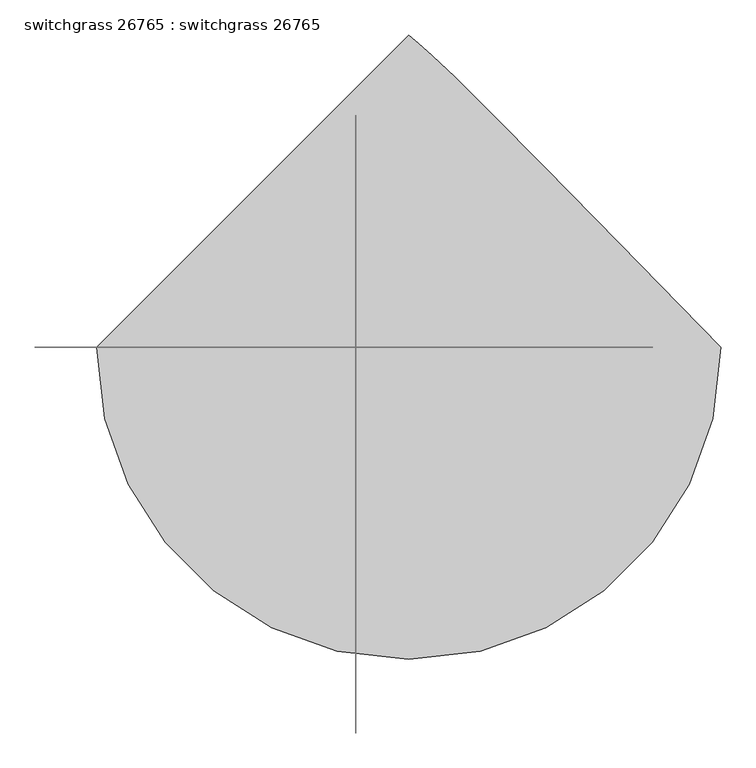
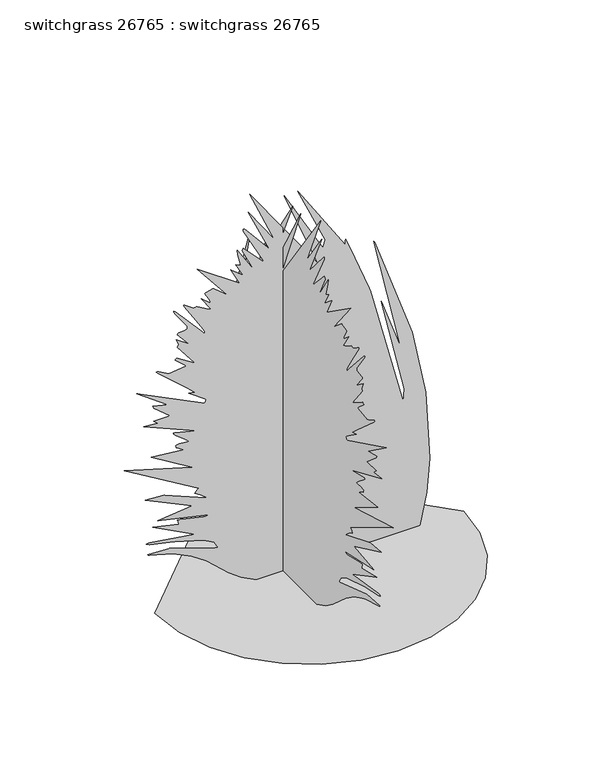
"""IFC4 building model written with IfcOpenShell, lengths in millimetres: proxy geometry, switchgrass 26765 : switchgrass 26765."""

import ifcopenshell
import ifcopenshell.guid

model = None  # the IFC model being written
_history = None  # IfcOwnerHistory: only IFC2X3 demands one
_inside = {}  # id of a spatial element -> (the spatial element, [elements in it])
_under = {}  # id of a project, library or spatial element -> (it, [spatial elements below it])
_declared = {}  # id of a project -> (the project, [libraries it declares])
_typed = {}  # id of a type object -> (the type object, [elements of that type])
_made_of = {}  # id of a material, layer set ... -> (it, [elements and type objects made of it])


def new_model(schema):
    """Start an empty IFC model of exactly this schema.

    Asked for "IFC4X3", IfcOpenShell would pick the latest addendum, in which some entities
    have other attributes; the version numbers below select the first issue.
    IFC2X3 requires an IfcOwnerHistory on every rooted entity: one is made here for all.
    """
    global model, _history
    if schema == "IFC4X3":
        model = ifcopenshell.file(schema_version=(4, 3, 0, 0))
    else:
        model = ifcopenshell.file(schema=schema)
    _inside.clear()
    _under.clear()
    _declared.clear()
    _typed.clear()
    _made_of.clear()
    _history = None
    if model.schema == "IFC2X3":
        org = make("IfcOrganization", Name="unknown")
        user = make(
            "IfcPersonAndOrganization",
            ThePerson=make("IfcPerson", FamilyName="unknown"),
            TheOrganization=org,
        )
        app = make(
            "IfcApplication",
            ApplicationDeveloper=org,
            Version="unknown",
            ApplicationFullName="unknown",
            ApplicationIdentifier="unknown",
        )
        _history = make(
            "IfcOwnerHistory",
            OwningUser=user,
            OwningApplication=app,
            ChangeAction="ADDED",
            CreationDate=0,
        )
    return model


def make(cls, **values):
    """One entity of the class cls with the attributes given. An attribute that is None is left unset."""
    return model.create_entity(
        cls, **{name: value for name, value in values.items() if value is not None}
    )


def rooted(cls, **values):
    """An entity with a GlobalId (a new one), such as an element, a storey or a relation."""
    return make(cls, GlobalId=ifcopenshell.guid.new(), OwnerHistory=_history, **values)


def si_unit(unit_type, name, prefix=None):
    """IfcSIUnit, for example si_unit("LENGTHUNIT", "METRE", prefix="MILLI")."""
    return make("IfcSIUnit", UnitType=unit_type, Prefix=prefix, Name=name)


def assignment(units):
    """IfcUnitAssignment: the units of a project."""
    return None if units is None else make("IfcUnitAssignment", Units=units)


def point(xyz):
    """IfcCartesianPoint."""
    return None if xyz is None else make("IfcCartesianPoint", Coordinates=xyz)


def direction(xyz):
    """IfcDirection."""
    return None if xyz is None else make("IfcDirection", DirectionRatios=xyz)


def frame(location, z_axis=None, x_axis=None):
    """IfcAxis2Placement3D, a coordinate frame: its origin and axes. An axis left out is left unset."""
    return make(
        "IfcAxis2Placement3D",
        Location=point(location),
        Axis=direction(z_axis),
        RefDirection=direction(x_axis),
    )


def origin():
    """The frame at (0, 0, 0) with its axes left unset."""
    return frame((0.0, 0.0, 0.0))


def place(relative_to, where):
    """IfcLocalPlacement: puts the frame where relative to a parent placement (None: the world)."""
    return make(
        "IfcLocalPlacement", PlacementRelTo=relative_to, RelativePlacement=where
    )


def context(
    kind, dimensions, precision=None, world=None, true_north=None, identifier=None
):
    """IfcGeometricRepresentationContext, for example the 3D "Model" context."""
    return make(
        "IfcGeometricRepresentationContext",
        ContextIdentifier=identifier,
        ContextType=kind,
        CoordinateSpaceDimension=dimensions,
        Precision=precision,
        WorldCoordinateSystem=world,
        TrueNorth=true_north,
    )


def project(units=None, contexts=None):
    """IfcProject with its units and contexts."""
    return rooted(
        "IfcProject",
        Name="project",
        RepresentationContexts=contexts,
        UnitsInContext=assignment(units),
    )


def spatial(cls, under=None, at=None, **own):
    """A site, building, storey or space (cls), placed at a placement, below another one or the project."""
    s = rooted(cls, ObjectPlacement=at, **own)
    if under is not None:
        _under.setdefault(under.id(), (under, []))[1].append(s)
    return s


def point_list(points):
    """IfcCartesianPointList2D or 3D."""
    cls = (
        "IfcCartesianPointList2D" if len(points[0]) == 2 else "IfcCartesianPointList3D"
    )
    return make(cls, CoordList=points)


def triangles(points, corners, closed=None, point_numbers=None):
    """IfcTriangulatedFaceSet: each triangle names its three corners, points numbered from 1."""
    return make(
        "IfcTriangulatedFaceSet",
        Coordinates=point_list(points),
        Closed=closed,
        CoordIndex=corners,
        PnIndex=point_numbers,
    )


def shape(context_of_items, identifier, shape_type, items):
    """IfcShapeRepresentation: the items that make up one representation, for example the "Body"."""
    return make(
        "IfcShapeRepresentation",
        ContextOfItems=context_of_items,
        RepresentationIdentifier=identifier,
        RepresentationType=shape_type,
        Items=items,
    )


def source(mapping_origin, context_of_items, identifier, shape_type, items):
    """IfcRepresentationMap: a shape defined once, which mapped items show again and again."""
    return make(
        "IfcRepresentationMap",
        MappingOrigin=mapping_origin,
        MappedRepresentation=shape(context_of_items, identifier, shape_type, items),
    )


def transform(
    local_origin,
    x_axis=None,
    y_axis=None,
    z_axis=None,
    scale=None,
    scale2=None,
    scale3=None,
    uniform=True,
):
    """IfcCartesianTransformationOperator3D, or its non-uniform kind. x_axis, y_axis, z_axis: its Axis1, 2, 3."""
    if uniform:
        return make(
            "IfcCartesianTransformationOperator3D",
            Axis1=direction(x_axis),
            Axis2=direction(y_axis),
            LocalOrigin=point(local_origin),
            Scale=scale,
            Axis3=direction(z_axis),
        )
    return make(
        "IfcCartesianTransformationOperator3DnonUniform",
        Axis1=direction(x_axis),
        Axis2=direction(y_axis),
        LocalOrigin=point(local_origin),
        Scale=scale,
        Axis3=direction(z_axis),
        Scale2=scale2,
        Scale3=scale3,
    )


def mapped(mapping_source, mapping_target):
    """IfcMappedItem: shows the shape of a source again, moved by a transform."""
    return make(
        "IfcMappedItem", MappingSource=mapping_source, MappingTarget=mapping_target
    )


def made_of(thing, what):
    """Note that an element or type object is made of a material, layer set ...; save() writes the relation."""
    if what is not None:
        _made_of.setdefault(what.id(), (what, []))[1].append(thing)
    return thing


def element(
    cls,
    number,
    at=None,
    inside=None,
    cuts=None,
    type_object=None,
    material=None,
    context=None,
    identifier="Body",
    shape_type=None,
    held_by="IfcProductDefinitionShape",
    body=None,
    shapes=None,
    **own,
):
    """One element of the class cls, such as IfcWall. Its Tag is "e" and its number.

    at: its placement. inside: the storey or other place that contains it. cuts: it is an
    opening in that element (IfcRelVoidsElement). A single representation is given by context,
    identifier, shape_type and body (its items); several are given by shapes. held_by: the class
    of the entity that holds the representations. save() writes the other relations.
    """
    e = rooted(cls, Tag="e%d" % number, ObjectPlacement=at, **own)
    if body is not None:
        shapes = [shape(context, identifier, shape_type, body)]
    if shapes is not None:
        e.Representation = make(held_by, Representations=shapes)
    if inside is not None:
        _inside.setdefault(inside.id(), (inside, []))[1].append(e)
    if cuts is not None:
        rooted(
            "IfcRelVoidsElement", RelatingBuildingElement=cuts, RelatedOpeningElement=e
        )
    if type_object is not None:
        _typed.setdefault(type_object.id(), (type_object, []))[1].append(e)
    return made_of(e, material)


def aggregate(whole, parts):
    """IfcRelAggregates: a whole, such as a stair, and the parts it consists of."""
    return rooted("IfcRelAggregates", RelatingObject=whole, RelatedObjects=parts)


def save(model, path):
    """Write the relations noted so far, then the file.

    IfcRelAggregates (storeys below a building ...), IfcRelContainedInSpatialStructure (elements
    in a storey), IfcRelDefinesByType, IfcRelAssociatesMaterial and IfcRelDeclares: one each for
    every whole, place, type object, material and project.
    """
    for whole, parts in _under.values():
        aggregate(whole, parts)
    for where, things in _inside.values():
        rooted(
            "IfcRelContainedInSpatialStructure",
            RelatedElements=things,
            RelatingStructure=where,
        )
    for kind, things in _typed.values():
        rooted("IfcRelDefinesByType", RelatedObjects=things, RelatingType=kind)
    for what, things in _made_of.values():
        rooted("IfcRelAssociatesMaterial", RelatedObjects=things, RelatingMaterial=what)
    for by, libraries in _declared.values():
        rooted("IfcRelDeclares", RelatingContext=by, RelatedDefinitions=libraries)
    model.write(path)


def switchgrass_26765_switchgrass_26765_d4ad6bd8(model_context):
    return source(origin(), model_context, "Body", "Tessellation", [
        triangles([(-459.698612, 0.0, 4.65e-05), (-447.5447391, -105.3326149, 4.65e-05), (-412.9347513, -202.0637927, 4.65e-05), (-358.6347227, -287.4208646, 4.65e-05), (-287.4208646, -358.6372662, 4.65e-05), (-202.0637927, -412.9347513, 4.65e-05), (-105.3326149, -447.5447391, 4.65e-05), (2.01e-05, -459.698612, 4.65e-05), (105.3326149, -447.5447391, 4.65e-05), (202.0637927, -412.9347513, 4.65e-05), (287.4208646, -358.6347227, 4.65e-05), (358.6372662, -287.4208646, 4.65e-05), (412.9347513, -202.0637927, 4.65e-05), (447.5447391, -105.3326149, 4.65e-05), (459.698612, 4.02e-05, 4.65e-05), (310.3062409, 153.2394836, 4.65e-05), (199.5550432, 266.0620302, 4.65e-05), (121.0036242, 345.2057822, 4.65e-05), (68.212606, 397.4052123, 4.65e-05), (34.7415567, 429.3964645, 4.65e-05), (14.1507237, 447.915574, 4.65e-05), (-6.03e-05, 459.698612, 4.65e-05), (25.778164, 7.09e-05, 931.0228226), (-73.9743319, 5.62e-05, 1178.5581493), (40.5563681, 6.83e-05, 975.3584158), (47.9454701, 6.69e-05, 997.5250134), (-33.3343979, 5.62e-05, 1178.5581493), (107.0580365, 6.91e-05, 960.5807568), (108.009768, 6.88e-05, 974.8428223), (108.4339518, 6.88e-05, 976.8163937), (108.9381361, 6.87e-05, 977.5631504), (121.537794, 7.04e-05, 948.2515675), (179.4161744, 7.78e-05, 798.7728281), (181.6249422, 7.82e-05, 791.64056), (280.7025792, 0.0001022, 406.3993581), (283.3568685, 9.98e-05, 447.039283), (214.1996435, 8.19e-05, 746.2965254), (273.311188, 9.18e-05, 580.0436282), (192.0325918, 7.02e-05, 942.1073204), (195.7270065, 7.05e-05, 938.4116884), (306.5800512, 8.97e-05, 615.8245474), (346.866909, 0.0001017, 413.7119931), (359.1935185, 0.0001144, 200.6111561), (350.2374882, 0.0001206, 97.2772745), (328.7313518, 0.0001264, 3.02e-05), (-155.9468584, 0.0001256, 0.034436), (-202.0081638, 0.0001242, 22.9207712), (-238.8497922, 0.0001227, 50.4692123), (-306.8086347, 0.0001194, 111.5848133), (-348.8913131, 0.0001178, 141.1673826), (-403.686624, 0.0001164, 167.4436493), (-477.2830038, 0.0001152, 188.5593844), (-477.9662833, 0.0001151, 188.9317636), (-478.6673306, 0.0001151, 189.4758256), (-479.3200888, 0.0001151, 190.1286019), (-479.8636602, 0.000115, 190.8281231), (-480.2344952, 0.000115, 191.5116207), (-480.3742032, 0.000115, 192.1161441), (-413.8720124, 0.0001152, 188.421475), (-269.7856765, 0.000118, 140.3924299), (-282.1148113, 0.0001168, 160.9176305), (-313.8012674, 0.0001157, 178.5812689), (-403.4097877, 0.0001139, 205.4826247), (-474.9589087, 0.000113, 221.4147554), (-484.0673281, 0.000113, 225.3669851), (-481.6365535, 0.000113, 227.0964581), (-478.1059914, 0.0001131, 227.7690551), (-473.780347, 0.0001131, 227.6730399), (-339.9809921, 0.0001141, 206.8940938), (-465.5965078, 0.0001101, 273.3949947), (-388.0097829, 0.0001112, 254.9241563), (-391.5657795, 0.0001104, 268.675697), (-391.7054875, 0.0001103, 269.7018517), (-378.6955985, 0.0001105, 267.1821653), (-313.5091704, 0.0001114, 252.3912622), (-310.4256014, 0.0001114, 251.228706), (-299.3410672, 0.0001112, 254.9241563), (-450.816269, 0.0001092, 288.1752335), (-347.369858, 0.0001086, 299.2572424), (-487.7630327, 0.0001046, 365.7593968), (-432.3454124, 0.0001048, 362.0637285), (-306.7298967, 0.0001079, 310.3417766), (-306.6994117, 0.0001078, 311.3857172), (-309.3435817, 0.0001077, 314.1746458), (-314.0120831, 0.0001074, 318.1928962), (-320.0598244, 0.0001072, 322.9223677), (-333.6919501, 0.0001066, 332.4448242), (-339.9809921, 0.0001064, 336.2040061), (-339.5619043, 0.0001063, 337.0523918), (-332.7115231, 0.0001059, 344.2304057), (-328.896458, 0.0001057, 347.2860332), (-550.5695189, 9.78e-05, 480.2903784), (-347.369858, 0.0001013, 421.1770535), (-469.2896327, 9.69e-05, 495.0680737), (-373.2320875, 9.76e-05, 483.9835396), (-374.0728065, 9.75e-05, 484.9741405), (-391.8451592, 9.68e-05, 496.840967), (-395.3986124, 9.67e-05, 498.7637784), (-395.5967471, 9.66e-05, 499.9347098), (-396.9810376, 9.65e-05, 504.0037565), (-397.0470946, 9.64e-05, 505.1086673), (-396.5848045, 9.63e-05, 505.8681413), (-395.3986124, 9.62e-05, 506.1526079), (-391.824848, 9.63e-05, 507.3895964), (-386.3283085, 9.63e-05, 507.7426635), (-361.3779056, 9.63e-05, 505.9697339), (-358.4543921, 9.62e-05, 506.1526079), (-365.3428525, 9.57e-05, 513.0766402), (-398.2154826, 9.31e-05, 538.6416859), (-403.0567205, 9.28e-05, 543.2873689), (-404.6620005, 9.27e-05, 546.7493669), (-400.0315782, 9.31e-05, 546.74428), (-336.2878309, 9.47e-05, 532.0148375), (-491.4561939, 9.07e-05, 598.5144848), (-450.816269, 9.09e-05, 594.8213236), (-458.7029606, 9.05e-05, 601.7732975), (-461.4817154, 9.03e-05, 605.0168859), (-461.9008032, 9.03e-05, 605.9033143), (-413.8720124, 9.03e-05, 605.9033143), (-461.9008032, 8.79e-05, 646.5432392), (-465.5965078, 8.74e-05, 653.9346485), (-421.2608783, 8.81e-05, 642.850078), (-513.6252623, 8.41e-05, 709.3522688), (-310.4256014, 9.01e-05, 609.599019), (-306.7298967, 8.94e-05, 620.6835531), (-358.4543921, 8.72e-05, 657.6278097), (-339.9809921, 8.74e-05, 653.9346485), (-364.4437068, 8.67e-05, 676.0859854), (-450.3971449, 8.26e-05, 751.897201), (-454.5119373, 8.13e-05, 757.3810959), (-451.4106005, 8.15e-05, 757.7264963), (-446.9833998, 8.18e-05, 756.2457001), (-417.5677171, 8.24e-05, 738.9076595), (-367.3392786, 8.19e-05, 745.9485815), (-365.8432217, 8.19e-05, 746.2965254), (-399.0943171, 8.02e-05, 775.8519161), (-398.8123939, 8.01e-05, 776.4208494), (-398.0529199, 8.01e-05, 777.091448), (-396.9480091, 8e-05, 777.7924953), (-394.2302244, 8e-05, 779.0167665), (-392.876419, 7.99e-05, 779.4028622), (-391.7054875, 7.99e-05, 779.5476208), (-342.833398, 8.18e-05, 747.6173023), (-339.9809921, 8.19e-05, 746.2965254), (-391.7054875, 7.8e-05, 812.7987162), (-388.0097829, 7.75e-05, 820.187582), (-395.3986124, 7.64e-05, 838.6609457), (-358.4543921, 7.8e-05, 812.7987162), (-391.7054875, 7.55e-05, 853.4386047), (-391.1365179, 7.55e-05, 854.4724079), (-390.4684991, 7.54e-05, 855.4528713), (-389.7649083, 7.54e-05, 856.3113945), (-389.0994329, 7.53e-05, 856.9742901), (-388.5406371, 7.53e-05, 857.3807333), (-388.1545415, 7.53e-05, 857.454348), (-388.0097829, 7.53e-05, 857.1343094), (-371.4439336, 7.53e-05, 857.9572969), (-366.4147347, 7.52e-05, 859.1713943), (-363.3692811, 7.51e-05, 861.0890825), (-362.1704081, 7.49e-05, 863.8297583), (-362.6758641, 7.47e-05, 867.5178326), (-364.7484847, 7.44e-05, 872.2777891), (-398.1672297, 7.28e-05, 919.6461914), (-402.3683905, 7.2e-05, 927.1721855), (-402.7874783, 7.09e-05, 931.0228226), (-397.8573286, 7.11e-05, 927.2000908), (-324.6191028, 7.61e-05, 844.1930208), (-310.4256014, 7.71e-05, 827.5763752), (-310.4256014, 7.78e-05, 835.1430645), (-320.710039, 7.69e-05, 852.757905), (-345.0991027, 7.52e-05, 891.1626829), (-371.9874687, 7.2e-05, 934.0708197), (-373.2320875, 7.05e-05, 938.4116884), (-370.2628284, 7.08e-05, 937.8046034), (-365.6527173, 7.1e-05, 935.328083), (-343.6766968, 7.16e-05, 919.9407955), (-341.8986803, 7.15e-05, 920.3700571), (-337.7610332, 7.15e-05, 920.8247532), (-335.7900052, 7.15e-05, 920.8373978), (-334.1441028, 7.15e-05, 920.6977261), (-333.0112504, 7.15e-05, 920.4005785), (-332.5921626, 7.16e-05, 919.9407955), (-299.1302334, 7.27e-05, 900.3193188), (-294.3855376, 7.29e-05, 898.213706), (-291.9522195, 7.29e-05, 897.7717272), (-321.5075921, 7.02e-05, 942.1073204), (-295.647906, 7.16e-05, 919.9407955), (-294.9392465, 7.14e-05, 922.478286), (-296.4556329, 7.11e-05, 927.3702839), (-299.4274173, 7.08e-05, 933.6441015), (-310.4256014, 6.96e-05, 953.1918909), (-307.5325367, 6.95e-05, 954.7641787), (-286.1407102, 6.92e-05, 960.3648542), (-284.5633718, 6.91e-05, 960.5807568), (-243.9231744, 7.11e-05, 927.3296614), (-332.5921626, 6.45e-05, 1038.1649019), (-206.9776643, 6.98e-05, 949.4961863), (-232.8394033, 6.67e-05, 1001.2206453), (-231.0110992, 6.68e-05, 1000.0979668), (-195.8941475, 6.85e-05, 971.6627111), (-218.0614536, 6.61e-05, 1012.3026724), (-203.2832495, 6.65e-05, 1004.9138065), (-212.5006375, 6.44e-05, 1040.9334829), (-214.4800588, 6.35e-05, 1054.5479136), (-214.3667663, 6.34e-05, 1056.6383383), (-162.6433064, 6.83e-05, 975.3584158), (-199.5885623, 6.39e-05, 1049.2494724), (-195.8941475, 6.34e-05, 1056.6383383), (-136.7815765, 6.72e-05, 993.8318521), (-136.7815765, 6.77e-05, 997.1490915), (-195.320854, 6.02e-05, 1109.0105049), (-195.8941475, 5.99e-05, 1115.7516632), (-191.8857621, 6.01e-05, 1114.2327152), (-118.3086943, 6.52e-05, 1027.0829475), (-181.1159253, 5.7e-05, 1163.7804176), (-103.5307446, 6.36e-05, 1052.9426336), (-177.4215105, 5.37e-05, 1219.1980379), (-77.7843237, 7.9038071, 931.0228226), (-77.7843237, -91.8487905, 1178.5581493), (-77.7843237, 22.6819595, 975.3584158), (-77.7843237, 30.0710115, 997.5250134), (-77.7843237, -51.2088565, 1178.5581493), (-77.7843237, 89.1835734, 960.5807568), (-77.7843237, 90.1355684, 974.8428223), (-77.7843237, 90.5594887, 976.8163937), (-77.7843237, 91.0636821, 977.5631504), (-77.7843237, 103.6633309, 948.2515675), (-77.7843237, 161.5417022, 798.7728281), (-77.7843237, 163.7507425, 791.64056), (-77.7843237, 262.8260722, 406.3993581), (-77.7843237, 265.4829231, 447.039283), (-77.7843237, 196.3254257, 746.2965254), (-77.7843237, 255.4372245, 580.0436282), (-77.7843237, 174.1581196, 942.1073204), (-77.7843237, 177.8525525, 938.4116884), (-77.7843237, 288.7035625, 615.8245474), (-77.7843237, 328.9929637, 413.7119931), (-77.7843237, 341.3195732, 200.6111561), (-77.7843237, 332.3635428, 97.2772745), (-77.7843237, 310.854863, 0.0), (-77.7843237, -173.8213124, 0.0344058), (-77.7843237, -219.8826179, 22.9207462), (-77.7843237, -256.7250093, 50.4692123), (-77.7843237, -324.6826163, 111.5848133), (-77.7843237, -366.7652584, 141.1673826), (-77.7843237, -421.5605693, 167.4436493), (-77.7843237, -495.1569855, 188.5593844), (-77.7843237, -495.8402287, 188.9317636), (-77.7843237, -496.541276, 189.4758256), (-77.7843237, -497.1940341, 190.1286019), (-77.7843237, -497.7376056, 190.8281231), (-77.7843237, -498.1109839, 191.5113845), (-77.7843237, -498.2481485, 192.1161441), (-77.7843237, -431.7459578, 188.421475), (-77.7843237, -287.6596218, 140.3924299), (-77.7843237, -299.9887566, 160.9176305), (-77.7843237, -331.6752128, 178.5812689), (-77.7843237, -421.283733, 205.4826247), (-77.7843237, -492.8328541, 221.4147554), (-77.7843237, -501.9438532, 225.3669851), (-77.7843237, -499.5105351, 227.0964581), (-77.7843237, -495.9824801, 227.7690551), (-77.7843237, -491.6543286, 227.6730399), (-77.7843237, -357.8549375, 206.8940938), (-77.7843237, -483.4704532, 273.3949947), (-77.7843237, -405.8837282, 254.9241563), (-77.7843237, -409.4422683, 268.675697), (-77.7843237, -409.5794329, 269.7018517), (-77.7843237, -396.5695802, 267.1821653), (-77.7843237, -331.3831158, 252.3912622), (-77.7843237, -328.2995467, 251.228706), (-77.7843237, -317.2150126, 254.9241563), (-77.7843237, -468.6927578, 288.1752335), (-77.7843237, -365.2438033, 299.2572424), (-77.7843237, -505.6369781, 365.7593968), (-77.7843237, -450.2193578, 362.0637285), (-77.7843237, -324.6038784, 310.3417766), (-77.7843237, -324.5733933, 311.3857172), (-77.7843237, -327.217527, 314.1746458), (-77.7843237, -331.8885718, 318.1928962), (-77.7843237, -337.9337697, 322.9223677), (-77.7843237, -351.5659318, 332.4448242), (-77.7843237, -357.8549375, 336.2040061), (-77.7843237, -357.4358497, 337.0523918), (-77.7843237, -350.5854684, 344.2304057), (-77.7843237, -346.7729467, 347.2860332), (-77.7843237, -568.4434642, 480.2903784), (-77.7843237, -365.2438033, 421.1770535), (-77.7843237, -487.1636144, 495.0680737), (-77.7843237, -391.1060328, 483.9835396), (-77.7843237, -391.9467882, 484.9741405), (-77.7843237, -409.7191409, 496.840967), (-77.7843237, -413.2725941, 498.7637784), (-77.7843237, -413.4706924, 499.9347098), (-77.7843237, -414.8549829, 504.0037565), (-77.7843237, -414.92104, 505.1086673), (-77.7843237, -414.4587499, 505.8681413), (-77.7843237, -413.2725941, 506.1526079), (-77.7843237, -409.6987933, 507.3895964), (-77.7843237, -404.2022538, 507.7426635), (-77.7843237, -379.2518872, 505.9697339), (-77.7843237, -376.3283375, 506.1526079), (-77.7843237, -383.2167978, 513.0766402), (-77.7843237, -416.0894279, 538.6416859), (-77.7843237, -420.9306659, 543.2873689), (-77.7843237, -422.5359458, 546.7493669), (-77.7843237, -417.9055235, 546.74428), (-77.7843237, -354.1617763, 532.0148375), (-77.7843237, -509.3326827, 598.5144848), (-77.7843237, -468.6927578, 594.8213236), (-77.7843237, -476.5769059, 601.7732975), (-77.7843237, -479.3556607, 605.0168859), (-77.7843237, -479.7747485, 605.9033143), (-77.7843237, -431.7459578, 605.9033143), (-77.7843237, -479.7747485, 646.5432392), (-77.7843237, -483.4704532, 653.9346485), (-77.7843237, -439.1348236, 642.850078), (-77.7843237, -531.4992439, 709.3522688), (-77.7843237, -328.2995467, 609.599019), (-77.7843237, -324.6038784, 620.6835531), (-77.7843237, -376.3283375, 657.6278097), (-77.7843237, -357.8549375, 653.9346485), (-77.7843237, -382.3176521, 676.0859854), (-77.7843237, -468.2711266, 751.897201), (-77.7843237, -472.385919, 757.3810959), (-77.7843237, -469.2845821, 757.7264963), (-77.7843237, -464.8573451, 756.2457001), (-77.7843237, -435.4416624, 738.9076595), (-77.7843237, -385.2132603, 745.9485815), (-77.7843237, -383.7172033, 746.2965254), (-77.7843237, -416.9682624, 775.8544596), (-77.7843237, -416.6863392, 776.4208494), (-77.7843237, -415.9268652, 777.091448), (-77.7843237, -414.8245342, 777.7924953), (-77.7843237, -412.1041698, 779.0167665), (-77.7843237, -410.7529078, 779.4028622), (-77.7843237, -409.5794329, 779.5476208), (-77.7843237, -360.7098867, 747.6173023), (-77.7843237, -357.8549375, 746.2965254), (-77.7843237, -409.5794329, 812.7987162), (-77.7843237, -405.8837282, 820.187582), (-77.7843237, -413.2725941, 838.6609457), (-77.7843237, -376.3283375, 812.7987162), (-77.7843237, -409.5794329, 853.4386047), (-77.7843237, -409.0104632, 854.4724079), (-77.7843237, -408.3424444, 855.4528713), (-77.7843237, -407.6413971, 856.3113945), (-77.7843237, -406.9759217, 856.9742901), (-77.7843237, -406.4145824, 857.3807333), (-77.7843237, -406.0285232, 857.454348), (-77.7843237, -405.8837282, 857.1343094), (-77.7843237, -389.3204224, 857.9572969), (-77.7843237, -384.2912235, 859.1713943), (-77.7843237, -381.2432264, 861.0890825), (-77.7843237, -380.0443534, 863.8297583), (-77.7843237, -380.5498095, 867.5178326), (-77.7843237, -382.62243, 872.2803326), (-77.7843237, -416.0411751, 919.6461914), (-77.7843237, -420.2423358, 927.1721855), (-77.7843237, -420.663967, 931.0228226), (-77.7843237, -415.7313103, 927.2000908), (-77.7843237, -342.4955915, 844.1930208), (-77.7843237, -328.2995467, 827.5763752), (-77.7843237, -328.2995467, 835.1430645), (-77.7843237, -338.5839844, 852.757905), (-77.7843237, -362.973048, 891.1626829), (-77.7843237, -389.8639938, 934.0708197), (-77.7843237, -391.1060328, 938.4116884), (-77.7843237, -388.1367737, 937.8046034), (-77.7843237, -383.526699, 935.328083), (-77.7843237, -361.5506421, 919.9407955), (-77.7843237, -359.772662, 920.3700571), (-77.7843237, -355.6375219, 920.8247532), (-77.7843237, -353.666494, 920.8373978), (-77.7843237, -352.0180481, 920.6977261), (-77.7843237, -350.8877392, 920.4005785), (-77.7843237, -350.4661079, 919.9407955), (-77.7843237, -317.0041969, 900.3193188), (-77.7843237, -312.2594647, 898.213706), (-77.7843237, -309.8261467, 897.7717272), (-77.7843237, -339.3815738, 942.1073204), (-77.7843237, -313.5218513, 919.9407955), (-77.7843237, -312.81321, 922.478286), (-77.7843237, -314.3295782, 927.3702839), (-77.7843237, -317.3013808, 933.6441015), (-77.7843237, -328.2995467, 953.1918909), (-77.7843237, -325.406482, 954.7641787), (-77.7843237, -304.0146555, 960.3648542), (-77.7843237, -302.4373172, 960.5807568), (-77.7843237, -261.7973741, 927.3296614), (-77.7843237, -350.4661079, 1038.1649019), (-77.7843237, -224.8521183, 949.4961863), (-77.7843237, -250.7138573, 1001.2206453), (-77.7843237, -248.8855714, 1000.0979668), (-77.7843237, -213.7686015, 971.6627111), (-77.7843237, -235.9356533, 1012.3026724), (-77.7843237, -221.1577035, 1004.9138065), (-77.7843237, -230.3750915, 1040.9334829), (-77.7843237, -232.3545128, 1054.5479136), (-77.7843237, -232.2412203, 1056.6383383), (-77.7843237, -180.5177605, 975.3584158), (-77.7843237, -217.4630163, 1049.2494724), (-77.7843237, -213.7686015, 1056.6383383), (-77.7843237, -154.6557853, 993.8318521), (-77.7843237, -154.6557853, 997.1490915), (-77.7843237, -213.1953262, 1109.0105049), (-77.7843237, -213.7686015, 1115.7516632), (-77.7843237, -209.7602343, 1114.2327152), (-77.7843237, -136.1831483, 1027.0829475), (-77.7843237, -198.9903975, 1163.7804176), (-77.7843237, -121.4049442, 1052.9426336), (-77.7843237, -195.2957102, 1219.1980379)], [[21, 22, 1], [20, 21, 1], [19, 20, 1], [18, 19, 1], [17, 18, 1], [17, 1, 2], [17, 2, 3], [17, 3, 4], [16, 17, 4], [16, 4, 5], [16, 5, 6], [16, 6, 7], [16, 7, 8], [16, 8, 9], [16, 9, 10], [16, 10, 11], [16, 11, 12], [15, 16, 12], [14, 15, 12], [13, 14, 12], [36, 37, 38], [23, 24, 25], [26, 27, 28], [122, 123, 124], [214, 215, 216], [216, 217, 23], [69, 70, 71], [91, 92, 93], [185, 186, 187], [195, 196, 197], [113, 114, 115], [77, 78, 79], [79, 80, 81], [79, 81, 82], [125, 126, 127], [93, 94, 95], [197, 198, 199], [38, 39, 40], [38, 40, 41], [146, 147, 148], [200, 201, 202], [204, 205, 206], [203, 204, 206], [202, 203, 206], [200, 202, 206], [164, 165, 166], [120, 121, 122], [119, 120, 122], [36, 38, 41], [36, 41, 42], [30, 31, 32], [29, 30, 32], [28, 29, 32], [77, 79, 82], [64, 65, 66], [64, 66, 67], [129, 130, 131], [197, 199, 200], [163, 164, 166], [129, 131, 132], [119, 122, 124], [64, 67, 68], [172, 173, 174], [211, 212, 213], [117, 118, 119], [116, 117, 119], [115, 116, 119], [113, 115, 119], [113, 119, 124], [110, 111, 112], [35, 36, 42], [207, 208, 209], [206, 207, 209], [72, 73, 74], [57, 58, 59], [56, 57, 59], [55, 56, 59], [54, 55, 59], [53, 54, 59], [52, 53, 59], [51, 52, 59], [51, 59, 60], [50, 51, 60], [49, 50, 60], [214, 216, 23], [25, 26, 28], [162, 163, 166], [162, 166, 167], [161, 162, 167], [160, 161, 167], [211, 213, 214], [210, 211, 214], [48, 49, 60], [172, 174, 175], [171, 172, 175], [190, 191, 192], [63, 64, 68], [63, 68, 69], [62, 63, 69], [109, 110, 112], [87, 88, 89], [129, 132, 133], [210, 214, 23], [209, 210, 23], [23, 25, 28], [108, 109, 112], [108, 112, 113], [107, 108, 113], [171, 175, 176], [44, 45, 46], [145, 146, 148], [144, 145, 148], [154, 155, 156], [135, 136, 137], [135, 137, 138], [135, 138, 139], [135, 139, 140], [135, 140, 141], [135, 141, 142], [135, 142, 143], [43, 44, 46], [171, 176, 177], [171, 177, 178], [171, 178, 179], [171, 179, 180], [171, 180, 181], [171, 181, 182], [171, 182, 183], [170, 171, 183], [170, 183, 184], [170, 184, 185], [42, 43, 46], [35, 42, 46], [35, 46, 47], [35, 47, 48], [35, 48, 60], [35, 60, 61], [34, 35, 61], [34, 61, 62], [34, 62, 69], [148, 149, 150], [148, 150, 151], [148, 151, 152], [148, 152, 153], [148, 153, 154], [148, 154, 156], [148, 156, 157], [148, 157, 158], [159, 160, 167], [148, 158, 159], [148, 159, 167], [148, 167, 168], [144, 148, 168], [128, 129, 133], [128, 133, 134], [128, 134, 135], [128, 135, 143], [128, 143, 144], [169, 170, 185], [71, 72, 74], [69, 71, 74], [69, 74, 75], [69, 75, 76], [23, 28, 32], [33, 34, 69], [197, 200, 206], [206, 209, 23], [190, 192, 193], [190, 193, 194], [190, 194, 195], [189, 190, 195], [188, 189, 195], [187, 188, 195], [185, 187, 195], [87, 89, 90], [87, 90, 91], [97, 98, 99], [127, 128, 144], [86, 87, 91], [23, 32, 33], [101, 102, 103], [100, 101, 103], [100, 103, 104], [99, 100, 104], [97, 99, 104], [97, 104, 105], [96, 97, 105], [96, 105, 106], [95, 96, 106], [95, 106, 107], [93, 95, 107], [93, 107, 113], [125, 127, 144], [197, 206, 23], [169, 185, 195], [69, 76, 77], [33, 69, 77], [33, 77, 82], [33, 82, 83], [33, 83, 84], [33, 84, 85], [33, 85, 86], [33, 86, 91], [33, 91, 93], [33, 93, 113], [33, 113, 124], [33, 124, 125], [33, 125, 144], [33, 144, 168], [23, 33, 168], [197, 23, 168], [195, 197, 168], [169, 195, 168], [231, 232, 233], [218, 219, 220], [221, 222, 223], [317, 318, 319], [409, 410, 411], [411, 412, 218], [264, 265, 266], [286, 287, 288], [380, 381, 382], [390, 391, 392], [308, 309, 310], [272, 273, 274], [274, 275, 276], [274, 276, 277], [320, 321, 322], [288, 289, 290], [392, 393, 394], [233, 234, 235], [233, 235, 236], [341, 342, 343], [395, 396, 397], [399, 400, 401], [398, 399, 401], [397, 398, 401], [395, 397, 401], [359, 360, 361], [315, 316, 317], [314, 315, 317], [231, 233, 236], [231, 236, 237], [225, 226, 227], [224, 225, 227], [223, 224, 227], [272, 274, 277], [259, 260, 261], [259, 261, 262], [324, 325, 326], [392, 394, 395], [358, 359, 361], [324, 326, 327], [314, 317, 319], [259, 262, 263], [367, 368, 369], [406, 407, 408], [312, 313, 314], [311, 312, 314], [310, 311, 314], [308, 310, 314], [308, 314, 319], [305, 306, 307], [230, 231, 237], [402, 403, 404], [401, 402, 404], [267, 268, 269], [252, 253, 254], [251, 252, 254], [250, 251, 254], [249, 250, 254], [248, 249, 254], [247, 248, 254], [246, 247, 254], [246, 254, 255], [245, 246, 255], [244, 245, 255], [409, 411, 218], [220, 221, 223], [357, 358, 361], [357, 361, 362], [356, 357, 362], [355, 356, 362], [406, 408, 409], [405, 406, 409], [243, 244, 255], [367, 369, 370], [366, 367, 370], [385, 386, 387], [258, 259, 263], [258, 263, 264], [257, 258, 264], [304, 305, 307], [282, 283, 284], [324, 327, 328], [405, 409, 218], [404, 405, 218], [218, 220, 223], [303, 304, 307], [303, 307, 308], [302, 303, 308], [366, 370, 371], [239, 240, 241], [340, 341, 343], [339, 340, 343], [349, 350, 351], [330, 331, 332], [330, 332, 333], [330, 333, 334], [330, 334, 335], [330, 335, 336], [330, 336, 337], [330, 337, 338], [238, 239, 241], [366, 371, 372], [366, 372, 373], [366, 373, 374], [366, 374, 375], [366, 375, 376], [366, 376, 377], [366, 377, 378], [365, 366, 378], [365, 378, 379], [365, 379, 380], [237, 238, 241], [230, 237, 241], [230, 241, 242], [230, 242, 243], [230, 243, 255], [230, 255, 256], [229, 230, 256], [229, 256, 257], [229, 257, 264], [343, 344, 345], [343, 345, 346], [343, 346, 347], [343, 347, 348], [343, 348, 349], [343, 349, 351], [343, 351, 352], [343, 352, 353], [354, 355, 362], [343, 353, 354], [343, 354, 362], [343, 362, 363], [339, 343, 363], [323, 324, 328], [323, 328, 329], [323, 329, 330], [323, 330, 338], [323, 338, 339], [364, 365, 380], [266, 267, 269], [264, 266, 269], [264, 269, 270], [264, 270, 271], [218, 223, 227], [228, 229, 264], [392, 395, 401], [401, 404, 218], [385, 387, 388], [385, 388, 389], [385, 389, 390], [384, 385, 390], [383, 384, 390], [382, 383, 390], [380, 382, 390], [282, 284, 285], [282, 285, 286], [292, 293, 294], [322, 323, 339], [281, 282, 286], [218, 227, 228], [296, 297, 298], [295, 296, 298], [295, 298, 299], [294, 295, 299], [292, 294, 299], [292, 299, 300], [291, 292, 300], [291, 300, 301], [290, 291, 301], [290, 301, 302], [288, 290, 302], [288, 302, 308], [320, 322, 339], [392, 401, 218], [364, 380, 390], [264, 271, 272], [228, 264, 272], [228, 272, 277], [228, 277, 278], [228, 278, 279], [228, 279, 280], [228, 280, 281], [228, 281, 286], [228, 286, 288], [228, 288, 308], [228, 308, 319], [228, 319, 320], [228, 320, 339], [228, 339, 363], [218, 228, 363], [392, 218, 363], [390, 392, 363], [364, 390, 363]], closed=False),
    ])


if __name__ == "__main__":
    model = new_model("IFC4")
    model_context = context("Model", 3, world=origin())
    ifc_project = project(units=[si_unit("LENGTHUNIT", "METRE", prefix="MILLI")], contexts=[model_context])
    site = spatial("IfcSite", under=ifc_project)
    building = spatial("IfcBuilding", under=site)
    placement = place(None, origin())
    switchgrass_26765_switchgrass_26765_shape = switchgrass_26765_switchgrass_26765_d4ad6bd8(model_context)
    element("IfcBuildingElementProxy", 1, Name="switchgrass 26765 : switchgrass 26765", ObjectType="switchgrass 26765 : switchgrass 26765", at=placement, inside=building, context=model_context, shape_type="MappedRepresentation", body=[
        mapped(switchgrass_26765_switchgrass_26765_shape, transform((0.0, 0.0, 0.0), x_axis=(1.0, 0.0, 0.0), y_axis=(0.0, 1.0, 0.0), z_axis=(0.0, 0.0, 1.0))),
    ])
    save(model, "model.ifc")

# Revit data of these elements
# Type "switchgrass 26765 : switchgrass 26765"
#   built-in parameter 1005195 = "RPC-16-FVP6-6SQ0-2RXK-S000-ST1L-LVER-AU"
#   Height = 0
